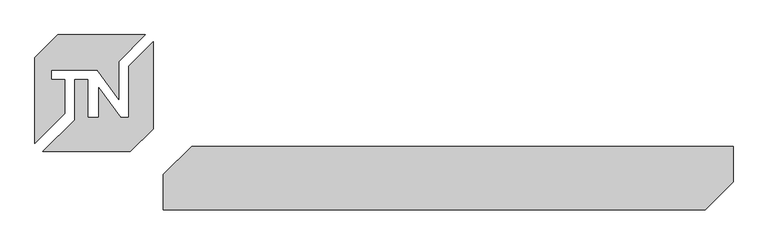
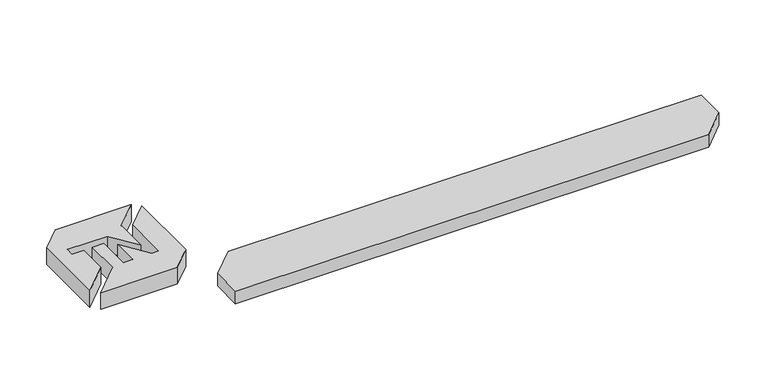
"""IFC4 building model written with IfcOpenShell, lengths in millimetres: proxy geometry, ТЕХНОНИКОЛЬ : ТЕХНОНИКОЛЬ."""

import ifcopenshell
import ifcopenshell.guid

model = None  # the IFC model being written
_history = None  # IfcOwnerHistory: only IFC2X3 demands one
_inside = {}  # id of a spatial element -> (the spatial element, [elements in it])
_under = {}  # id of a project, library or spatial element -> (it, [spatial elements below it])
_declared = {}  # id of a project -> (the project, [libraries it declares])
_typed = {}  # id of a type object -> (the type object, [elements of that type])
_made_of = {}  # id of a material, layer set ... -> (it, [elements and type objects made of it])


def new_model(schema):
    """Start an empty IFC model of exactly this schema.

    Asked for "IFC4X3", IfcOpenShell would pick the latest addendum, in which some entities
    have other attributes; the version numbers below select the first issue.
    IFC2X3 requires an IfcOwnerHistory on every rooted entity: one is made here for all.
    """
    global model, _history
    if schema == "IFC4X3":
        model = ifcopenshell.file(schema_version=(4, 3, 0, 0))
    else:
        model = ifcopenshell.file(schema=schema)
    _inside.clear()
    _under.clear()
    _declared.clear()
    _typed.clear()
    _made_of.clear()
    _history = None
    if model.schema == "IFC2X3":
        org = make("IfcOrganization", Name="unknown")
        user = make(
            "IfcPersonAndOrganization",
            ThePerson=make("IfcPerson", FamilyName="unknown"),
            TheOrganization=org,
        )
        app = make(
            "IfcApplication",
            ApplicationDeveloper=org,
            Version="unknown",
            ApplicationFullName="unknown",
            ApplicationIdentifier="unknown",
        )
        _history = make(
            "IfcOwnerHistory",
            OwningUser=user,
            OwningApplication=app,
            ChangeAction="ADDED",
            CreationDate=0,
        )
    return model


def make(cls, **values):
    """One entity of the class cls with the attributes given. An attribute that is None is left unset."""
    return model.create_entity(
        cls, **{name: value for name, value in values.items() if value is not None}
    )


def rooted(cls, **values):
    """An entity with a GlobalId (a new one), such as an element, a storey or a relation."""
    return make(cls, GlobalId=ifcopenshell.guid.new(), OwnerHistory=_history, **values)


def si_unit(unit_type, name, prefix=None):
    """IfcSIUnit, for example si_unit("LENGTHUNIT", "METRE", prefix="MILLI")."""
    return make("IfcSIUnit", UnitType=unit_type, Prefix=prefix, Name=name)


def assignment(units):
    """IfcUnitAssignment: the units of a project."""
    return None if units is None else make("IfcUnitAssignment", Units=units)


def point(xyz):
    """IfcCartesianPoint."""
    return None if xyz is None else make("IfcCartesianPoint", Coordinates=xyz)


def direction(xyz):
    """IfcDirection."""
    return None if xyz is None else make("IfcDirection", DirectionRatios=xyz)


def frame(location, z_axis=None, x_axis=None):
    """IfcAxis2Placement3D, a coordinate frame: its origin and axes. An axis left out is left unset."""
    return make(
        "IfcAxis2Placement3D",
        Location=point(location),
        Axis=direction(z_axis),
        RefDirection=direction(x_axis),
    )


def origin():
    """The frame at (0, 0, 0) with its axes left unset."""
    return frame((0.0, 0.0, 0.0))


def place(relative_to, where):
    """IfcLocalPlacement: puts the frame where relative to a parent placement (None: the world)."""
    return make(
        "IfcLocalPlacement", PlacementRelTo=relative_to, RelativePlacement=where
    )


def context(
    kind, dimensions, precision=None, world=None, true_north=None, identifier=None
):
    """IfcGeometricRepresentationContext, for example the 3D "Model" context."""
    return make(
        "IfcGeometricRepresentationContext",
        ContextIdentifier=identifier,
        ContextType=kind,
        CoordinateSpaceDimension=dimensions,
        Precision=precision,
        WorldCoordinateSystem=world,
        TrueNorth=true_north,
    )


def project(units=None, contexts=None):
    """IfcProject with its units and contexts."""
    return rooted(
        "IfcProject",
        Name="project",
        RepresentationContexts=contexts,
        UnitsInContext=assignment(units),
    )


def spatial(cls, under=None, at=None, **own):
    """A site, building, storey or space (cls), placed at a placement, below another one or the project."""
    s = rooted(cls, ObjectPlacement=at, **own)
    if under is not None:
        _under.setdefault(under.id(), (under, []))[1].append(s)
    return s


def polyline(points):
    """IfcPolyline through the points."""
    return make("IfcPolyline", Points=[point(p) for p in points])


def outline(outer, holes=None, kind="AREA"):
    """IfcArbitraryClosedProfileDef: a profile drawn as a closed curve; with holes, ...WithVoids."""
    if holes is None:
        return make("IfcArbitraryClosedProfileDef", ProfileType=kind, OuterCurve=outer)
    return make(
        "IfcArbitraryProfileDefWithVoids",
        ProfileType=kind,
        OuterCurve=outer,
        InnerCurves=holes,
    )


def extrude(swept, where, along, depth):
    """IfcExtrudedAreaSolid: the profile swept, set in the frame where, extruded along a direction by depth."""
    return make(
        "IfcExtrudedAreaSolid",
        SweptArea=swept,
        Position=where,
        ExtrudedDirection=direction(along),
        Depth=depth,
    )


def shape(context_of_items, identifier, shape_type, items):
    """IfcShapeRepresentation: the items that make up one representation, for example the "Body"."""
    return make(
        "IfcShapeRepresentation",
        ContextOfItems=context_of_items,
        RepresentationIdentifier=identifier,
        RepresentationType=shape_type,
        Items=items,
    )


def source(mapping_origin, context_of_items, identifier, shape_type, items):
    """IfcRepresentationMap: a shape defined once, which mapped items show again and again."""
    return make(
        "IfcRepresentationMap",
        MappingOrigin=mapping_origin,
        MappedRepresentation=shape(context_of_items, identifier, shape_type, items),
    )


def transform(
    local_origin,
    x_axis=None,
    y_axis=None,
    z_axis=None,
    scale=None,
    scale2=None,
    scale3=None,
    uniform=True,
):
    """IfcCartesianTransformationOperator3D, or its non-uniform kind. x_axis, y_axis, z_axis: its Axis1, 2, 3."""
    if uniform:
        return make(
            "IfcCartesianTransformationOperator3D",
            Axis1=direction(x_axis),
            Axis2=direction(y_axis),
            LocalOrigin=point(local_origin),
            Scale=scale,
            Axis3=direction(z_axis),
        )
    return make(
        "IfcCartesianTransformationOperator3DnonUniform",
        Axis1=direction(x_axis),
        Axis2=direction(y_axis),
        LocalOrigin=point(local_origin),
        Scale=scale,
        Axis3=direction(z_axis),
        Scale2=scale2,
        Scale3=scale3,
    )


def mapped(mapping_source, mapping_target):
    """IfcMappedItem: shows the shape of a source again, moved by a transform."""
    return make(
        "IfcMappedItem", MappingSource=mapping_source, MappingTarget=mapping_target
    )


def made_of(thing, what):
    """Note that an element or type object is made of a material, layer set ...; save() writes the relation."""
    if what is not None:
        _made_of.setdefault(what.id(), (what, []))[1].append(thing)
    return thing


def element(
    cls,
    number,
    at=None,
    inside=None,
    cuts=None,
    type_object=None,
    material=None,
    context=None,
    identifier="Body",
    shape_type=None,
    held_by="IfcProductDefinitionShape",
    body=None,
    shapes=None,
    **own,
):
    """One element of the class cls, such as IfcWall. Its Tag is "e" and its number.

    at: its placement. inside: the storey or other place that contains it. cuts: it is an
    opening in that element (IfcRelVoidsElement). A single representation is given by context,
    identifier, shape_type and body (its items); several are given by shapes. held_by: the class
    of the entity that holds the representations. save() writes the other relations.
    """
    e = rooted(cls, Tag="e%d" % number, ObjectPlacement=at, **own)
    if body is not None:
        shapes = [shape(context, identifier, shape_type, body)]
    if shapes is not None:
        e.Representation = make(held_by, Representations=shapes)
    if inside is not None:
        _inside.setdefault(inside.id(), (inside, []))[1].append(e)
    if cuts is not None:
        rooted(
            "IfcRelVoidsElement", RelatingBuildingElement=cuts, RelatedOpeningElement=e
        )
    if type_object is not None:
        _typed.setdefault(type_object.id(), (type_object, []))[1].append(e)
    return made_of(e, material)


def aggregate(whole, parts):
    """IfcRelAggregates: a whole, such as a stair, and the parts it consists of."""
    return rooted("IfcRelAggregates", RelatingObject=whole, RelatedObjects=parts)


def save(model, path):
    """Write the relations noted so far, then the file.

    IfcRelAggregates (storeys below a building ...), IfcRelContainedInSpatialStructure (elements
    in a storey), IfcRelDefinesByType, IfcRelAssociatesMaterial and IfcRelDeclares: one each for
    every whole, place, type object, material and project.
    """
    for whole, parts in _under.values():
        aggregate(whole, parts)
    for where, things in _inside.values():
        rooted(
            "IfcRelContainedInSpatialStructure",
            RelatedElements=things,
            RelatingStructure=where,
        )
    for kind, things in _typed.values():
        rooted("IfcRelDefinesByType", RelatedObjects=things, RelatingType=kind)
    for what, things in _made_of.values():
        rooted("IfcRelAssociatesMaterial", RelatedObjects=things, RelatingMaterial=what)
    for by, libraries in _declared.values():
        rooted("IfcRelDeclares", RelatingContext=by, RelatedDefinitions=libraries)
    model.write(path)


def generic_models_dc5aa90e(model_context):
    return source(origin(), model_context, "Body", "SweptSolid", [
        extrude(outline(polyline([(2060.18068, 6552.946455), (7456.1525037, 6552.946455), (7456.1525037, 6198.9182787), (7177.0333157, 5919.7990907), (1779.3758084, 5919.7990907), (1779.3758084, 6272.1415834), (2060.18068, 6552.946455)])), frame((0.0, 0.0, 4000.0), z_axis=(0.0, 0.0, 1.0), x_axis=(1.0, 0.0, 0.0)), (0.0, 0.0, 1.0), 150.0),
        extrude(outline(polyline([(500.0, 6582.0058801), (500.0, 7436.6570713), (729.7247093, 7666.3817806), (1599.7247093, 7666.3817806), (1334.4454033, 7401.1024746), (1334.4454033, 7021.1024746), (1122.8427125, 7312.3485926), (662.8427125, 7312.3485926), (662.8427125, 7219.8485926), (797.8427125, 7219.8485926), (797.8427125, 6879.8485926), (500.0, 6582.0058801)])), frame((0.0, 0.0, 4000.0), z_axis=(0.0, 0.0, 1.0), x_axis=(1.0, 0.0, 0.0)), (0.0, 0.0, 1.0), 200.0),
        extrude(outline(polyline([(898.1980515, 6818.4194782), (898.1980515, 7219.8485926), (1028.1980515, 7219.8485926), (1028.1980515, 6839.8485926), (1138.1980515, 6839.8485926), (1138.1980515, 7139.8485926), (1356.1608099, 6839.8485926), (1436.1608099, 6839.8485926), (1436.1608099, 7356.3822366), (1676.5771155, 7596.7985422), (1676.5771155, 6726.7985422), (1450.0, 6500.2214267), (580.0, 6500.2214267), (898.1980515, 6818.4194782)])), frame((0.0, 0.0, 4000.0), z_axis=(0.0, 0.0, 1.0), x_axis=(1.0, 0.0, 0.0)), (0.0, 0.0, 1.0), 200.0),
    ])


if __name__ == "__main__":
    model = new_model("IFC4")
    model_context = context("Model", 3, world=origin())
    ifc_project = project(units=[si_unit("LENGTHUNIT", "METRE", prefix="MILLI")], contexts=[model_context])
    site = spatial("IfcSite", under=ifc_project)
    building = spatial("IfcBuilding", under=site)
    placement = place(None, origin())
    generic_models_shape = generic_models_dc5aa90e(model_context)
    element("IfcBuildingElementProxy", 1, Name="ТЕХНОНИКОЛЬ : ТЕХНОНИКОЛЬ", ObjectType="ТЕХНОНИКОЛЬ : ТЕХНОНИКОЛЬ", at=placement, inside=building, context=model_context, shape_type="MappedRepresentation", body=[
        mapped(generic_models_shape, transform((0.0, 0.0, 0.0), x_axis=(1.0, 0.0, 0.0), y_axis=(0.0, 1.0, 0.0), z_axis=(0.0, 0.0, 1.0))),
    ])
    save(model, "model.ifc")

# Revit data of these elements
# Element 1 (IfcBuildingElementProxy, "ТЕХНОНИКОЛЬ : ТЕХНОНИКОЛЬ")
#   Materials on its faces: "TN_Логотип_ТехноНИКОЛЬ"
# Materials
#   "TN_Логотип_ТехноНИКОЛЬ": class "Типовые", colour RGB 255 0 0, transparency 0, Cost = 0
